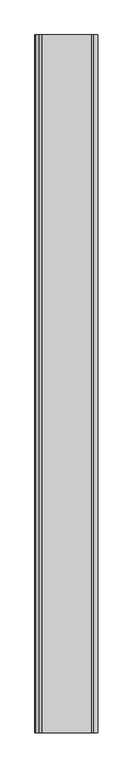
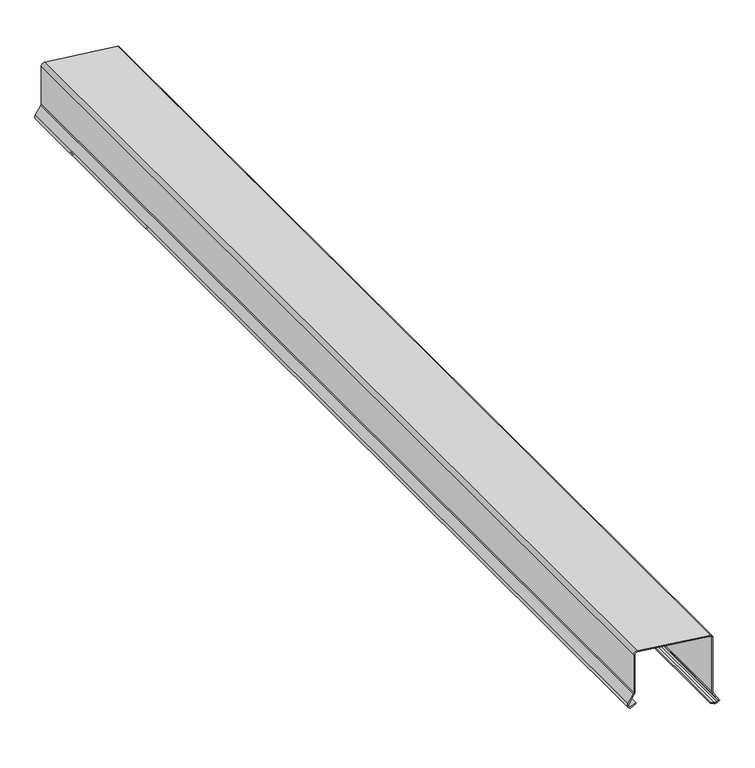
"""IFC4 building model written with IfcOpenShell, lengths in millimetres: proxy geometry, Flashing029 2285 : Flashing029 2285."""

from ifc_helpers import new_model, si_unit, point, frame, frame_2d, origin, place, context, project, spatial, polyline, circle_curve, trimmed, segment, composite_curve, outline, extrude, source, transform, mapped, element, save


def generic_models_23744907(model_context):
    return source(origin(), model_context, "Body", "SweptSolid", [
        extrude(outline(composite_curve([segment(polyline([(40086.398437, -7266.956055), (40092.152344, -7255.346191), (40093.9490864, -7256.2366656), (40088.6846745, -7266.8588577), (40089.8466166, -7268.7750305)]), True, "CONTINUOUS"), segment(trimmed(circle_curve(frame_2d((40093.4434175, -7266.287785)), 4.3730273), [point((40089.8466166, -7268.7750305))], [point((40095.7266973, -7270.0173964))], True, "CARTESIAN"), True, "CONTINUOUS"), segment(polyline([(40095.7266973, -7270.0173964), (40111.7309891, -7259.7605083)]), True, "CONTINUOUS"), segment(trimmed(circle_curve(frame_2d((40115.861873, -7265.806759)), 7.32266), [point((40111.7309891, -7259.7605083))], [point((40116.1385872, -7258.4893292))], False, "CARTESIAN"), True, "CONTINUOUS"), segment(polyline([(40116.1385872, -7258.4893292), (40193.276665, -7258.4893292)]), True, "CONTINUOUS"), segment(trimmed(circle_curve(frame_2d((40193.367253, -7254.1255777)), 4.3646917), [point((40193.276665, -7258.4893292))], [point((40197.6973721, -7253.5773062))], True, "CARTESIAN"), True, "CONTINUOUS"), segment(polyline([(40197.6973721, -7253.5773062), (40180.4916036, -7111.7967854)]), True, "CONTINUOUS"), segment(trimmed(circle_curve(frame_2d((40175.841451, -7112.759368)), 4.7487351), [point((40180.4916036, -7111.7967854))], [point((40175.9416385, -7108.0116899))], True, "CARTESIAN"), True, "CONTINUOUS"), segment(polyline([(40175.9416385, -7108.0116899), (40064.0437764, -7108.0116899)]), True, "CONTINUOUS"), segment(trimmed(circle_curve(frame_2d((40064.0983061, -7099.1269875)), 8.8848697), [point((40064.0437764, -7108.0116899))], [point((40059.2697952, -7106.5852979))], False, "CARTESIAN"), True, "CONTINUOUS"), segment(polyline([(40059.2697952, -7106.5852979), (40042.6162498, -7095.8037908), (40040.6845786, -7098.9401191)]), True, "CONTINUOUS"), segment(trimmed(circle_curve(frame_2d((40044.441402, -7101.272247)), 4.4218257), [point((40040.6845786, -7098.9401191))], [point((40040.4164008, -7103.1030686))], True, "CARTESIAN"), True, "CONTINUOUS"), segment(polyline([(40040.4164008, -7103.1030686), (40043.7762965, -7110.0176247), (40041.972656, -7110.894043), (40038.6026561, -7103.9586928)]), True, "CONTINUOUS"), segment(trimmed(circle_curve(frame_2d((40044.441402, -7101.272247)), 6.4271257), [point((40038.6026561, -7103.9586928))], [point((40038.9788223, -7097.8857786))], False, "CARTESIAN"), True, "CONTINUOUS"), segment(polyline([(40038.9788223, -7097.8857786), (40041.984375, -7093.005859), (40060.3595819, -7104.9019699)]), True, "CONTINUOUS"), segment(trimmed(circle_curve(frame_2d((40064.0983061, -7099.1269875)), 6.8795697), [point((40060.3595819, -7104.9019699))], [point((40064.0503229, -7106.0063899))], True, "CARTESIAN"), True, "CONTINUOUS"), segment(polyline([(40064.0503229, -7106.0063899), (40175.960936, -7106.0063899)]), True, "CONTINUOUS"), segment(trimmed(circle_curve(frame_2d((40175.841451, -7112.759368)), 6.7540351), [point((40175.960936, -7106.0063899))], [point((40182.4731108, -7111.4794937))], False, "CARTESIAN"), True, "CONTINUOUS"), segment(polyline([(40182.4731108, -7111.4794937), (40199.6874998, -7253.3310503)]), True, "CONTINUOUS"), segment(trimmed(circle_curve(frame_2d((40193.367253, -7254.1255777)), 6.3699917), [point((40199.6874998, -7253.3310503))], [point((40193.2578143, -7260.4946292))], False, "CARTESIAN"), True, "CONTINUOUS"), segment(polyline([(40193.2578143, -7260.4946292), (40116.0976578, -7260.4946292)]), True, "CONTINUOUS"), segment(trimmed(circle_curve(frame_2d((40115.861873, -7265.806759)), 5.31736), [point((40116.0976578, -7260.4946292))], [point((40112.8398424, -7261.4316421))], True, "CARTESIAN"), True, "CONTINUOUS"), segment(polyline([(40112.8398424, -7261.4316421), (40096.7929689, -7271.7158201)]), True, "CONTINUOUS"), segment(trimmed(circle_curve(frame_2d((40093.4434175, -7266.287785)), 6.3783273), [point((40096.7929689, -7271.7158201))], [point((40088.1601567, -7269.8613287))], False, "CARTESIAN"), True, "CONTINUOUS"), segment(polyline([(40088.1601567, -7269.8613287), (40086.398437, -7266.956055)]), True, "CONTINUOUS")], self_intersect=False)), frame((0.0, 7982.1531721, 0.0), z_axis=(0.0, 1.0, 0.0), x_axis=(0.0, 0.0, 1.0)), (0.0, 0.0, 1.0), 1999.85),
    ])


if __name__ == "__main__":
    model = new_model("IFC4")
    model_context = context("Model", 3, world=origin())
    ifc_project = project(units=[si_unit("LENGTHUNIT", "METRE", prefix="MILLI")], contexts=[model_context])
    site = spatial("IfcSite", under=ifc_project)
    building = spatial("IfcBuilding", under=site)
    placement = place(None, origin())
    generic_models_shape = generic_models_23744907(model_context)
    element("IfcBuildingElementProxy", 1, Name="Flashing029 2285 : Flashing029 2285", ObjectType="Flashing029 2285 : Flashing029 2285", at=placement, inside=building, context=model_context, shape_type="MappedRepresentation", body=[
        mapped(generic_models_shape, transform((0.0, 0.0, 0.0), x_axis=(1.0, 0.0, 0.0), y_axis=(0.0, 1.0, 0.0), z_axis=(0.0, 0.0, 1.0))),
    ])
    save(model, "model.ifc")

# Revit data of these elements
# Type "Flashing029 2285 : Flashing029 2285"
#   NameOverride = "Flashing029"
# Element 1 (IfcBuildingElementProxy, "Flashing029 2285 : Flashing029 2285")
#   Materials on its faces: "METAL COPING"
# Materials
#   "METAL COPING": class "Unassigned", colour RGB 128 128 128, transparency 0
